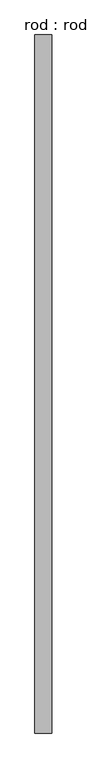
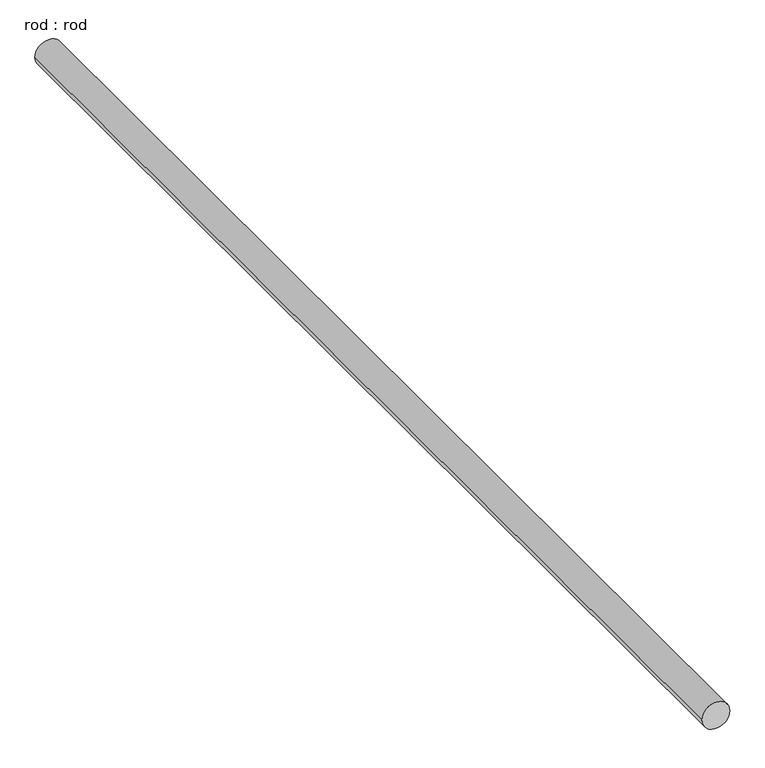
"""IFC4 building model written with IfcOpenShell, lengths in millimetres: proxy geometry, rod : rod."""

from ifc_helpers import new_model, si_unit, point, frame, frame_2d, origin, place, context, project, spatial, circle_curve, trimmed, segment, composite_curve, outline, extrude, source, transform, mapped, element, save


def rod_rod_28b0bef9(model_context):
    return source(origin(), model_context, "Body", "SweptSolid", [
        extrude(outline(composite_curve([segment(trimmed(circle_curve(frame_2d((0.0108462, 0.0)), 200.0), [point((0.0108462, 200.0))], [point((0.0108462, -200.0))], False, "CARTESIAN"), True, "CONTINUOUS"), segment(trimmed(circle_curve(frame_2d((0.0108462, 0.0)), 200.0), [point((0.0108462, -200.0))], [point((0.0108462, 200.0))], False, "CARTESIAN"), True, "CONTINUOUS")], self_intersect=False)), frame((0.0, -4207.2713847, 0.0), z_axis=(0.0, 1.0, 0.0), x_axis=(0.0, 0.0, 1.0)), (0.0, 0.0, 1.0), 16600.0),
    ])


if __name__ == "__main__":
    model = new_model("IFC4")
    model_context = context("Model", 3, world=origin())
    ifc_project = project(units=[si_unit("LENGTHUNIT", "METRE", prefix="MILLI")], contexts=[model_context])
    site = spatial("IfcSite", under=ifc_project)
    building = spatial("IfcBuilding", under=site)
    placement = place(None, origin())
    rod_rod_shape = rod_rod_28b0bef9(model_context)
    element("IfcBuildingElementProxy", 1, Name="rod : rod", ObjectType="rod : rod", at=placement, inside=building, context=model_context, shape_type="MappedRepresentation", body=[
        mapped(rod_rod_shape, transform((0.0, 0.0, 0.0), x_axis=(1.0, 0.0, 0.0), y_axis=(0.0, 1.0, 0.0), z_axis=(0.0, 0.0, 1.0))),
    ])
    save(model, "model.ifc")

# Revit data of these elements
# Type "rod : rod"
#   Default Elevation = 0
